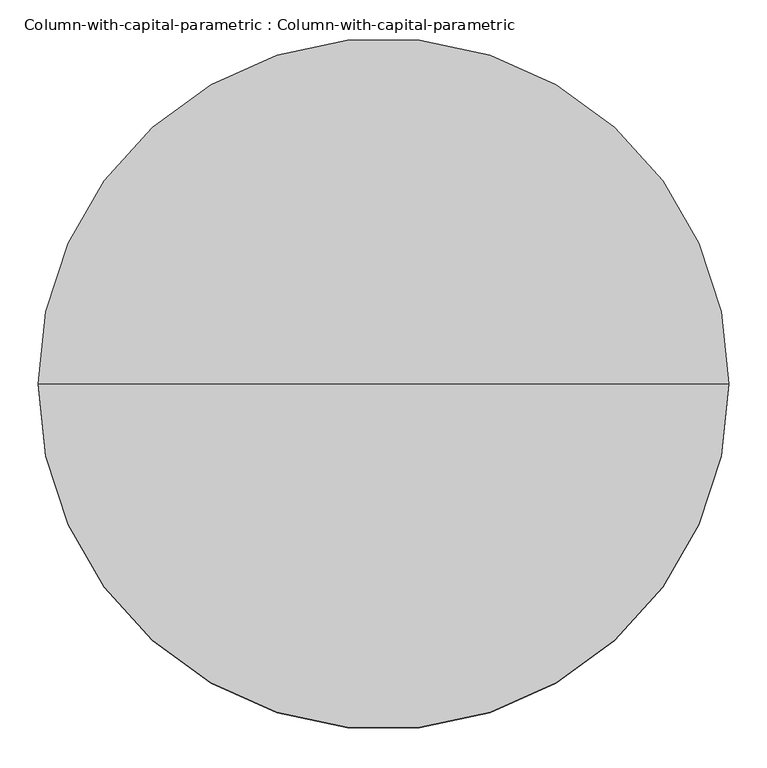
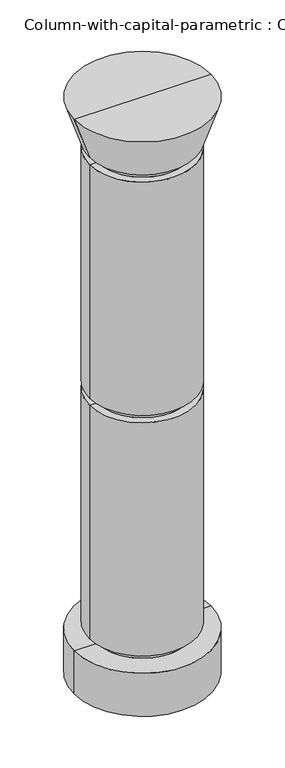
"""IFC4 building model written with IfcOpenShell, lengths in millimetres: column geometry, Column-with-capital-parametric : Column-with-capital-parametric."""

from ifc_helpers import new_model, si_unit, frame, origin, origin_with_axes, place, context, project, spatial, polyline, circle_curve, source, transform, mapped, element, save
from ifc_brep_helpers import plane_surface, cylinder_surface, revolved_surface, advanced_brep


def column_with_capital_parametric_column_with_capital_d26f2c8e(model_context):
    return source(origin(), model_context, "Body", "AdvancedBrep", [
        advanced_brep(
        [(-450.0, 0.0, 300.0), (450.0, 0.0, 300.0), (450.0, 0.0, 0.0), (-450.0, 0.0, 0.0), (0.0, 0.0, 0.0), (-300.0, 0.0, 300.0), (300.0, 0.0, 300.0), (-300.0, 0.0, 350.0), (300.0, 0.0, 350.0), (-350.0, 0.0, 350.0), (350.0, 0.0, 350.0), (-350.0, 0.0, 1975.0), (350.0, 0.0, 1975.0), (0.0, 0.0, 4000.0), (450.0, 0.0, 4000.0), (-450.0, 0.0, 4000.0), (350.0, 0.0, 3700.0), (-350.0, 0.0, 3700.0), (-300.0, 0.0, 3650.0), (300.0, 0.0, 3650.0), (350.0, 0.0, 3650.0), (-350.0, 0.0, 3650.0), (350.0, 0.0, 2025.0), (-350.0, 0.0, 2025.0), (-300.0, 0.0, 3700.0), (300.0, 0.0, 3700.0), (-300.0, 0.0, 1975.0), (300.0, 0.0, 1975.0), (-300.0, 0.0, 2025.0), (300.0, 0.0, 2025.0)],
        [
            (0, 1, circle_curve(frame((0.0, 0.0, 300.0), z_axis=(0.0, 0.0, -1.0), x_axis=(1.0, 0.0, 0.0)), 450.0)),
            (1, 2),
            (2, 3, circle_curve(origin_with_axes(), 450.0)),
            (3, 0),
            (2, 4),
            (4, 3),
            (2, 3, circle_curve(frame((0.0, 0.0, 0.0), z_axis=(0.0, 0.0, -1.0), x_axis=(1.0, 0.0, 0.0)), 450.0)),
            (1, 0, circle_curve(frame((0.0, 0.0, 300.0), z_axis=(0.0, 0.0, -1.0), x_axis=(1.0, 0.0, 0.0)), 450.0)),
            (5, 6, circle_curve(frame((0.0, 0.0, 300.0), z_axis=(0.0, 0.0, -1.0), x_axis=(1.0, 0.0, 0.0)), 300.0)),
            (6, 1),
            (0, 5),
            (6, 5, circle_curve(frame((0.0, 0.0, 300.0), z_axis=(0.0, 0.0, -1.0), x_axis=(1.0, 0.0, 0.0)), 300.0)),
            (7, 8, circle_curve(frame((0.0, 0.0, 350.0), z_axis=(0.0, 0.0, -1.0), x_axis=(1.0, 0.0, 0.0)), 300.0)),
            (8, 6),
            (5, 7),
            (8, 7, circle_curve(frame((0.0, 0.0, 350.0), z_axis=(0.0, 0.0, -1.0), x_axis=(1.0, 0.0, 0.0)), 300.0)),
            (9, 10, circle_curve(frame((0.0, 0.0, 350.0), z_axis=(0.0, 0.0, -1.0), x_axis=(1.0, 0.0, 0.0)), 350.0)),
            (10, 8),
            (7, 9),
            (10, 9, circle_curve(frame((0.0, 0.0, 350.0), z_axis=(0.0, 0.0, -1.0), x_axis=(1.0, 0.0, 0.0)), 350.0)),
            (11, 12, circle_curve(frame((0.0, 0.0, 1975.0), z_axis=(0.0, 0.0, -1.0), x_axis=(1.0, 0.0, 0.0)), 350.0)),
            (12, 10),
            (9, 11),
            (12, 11, circle_curve(frame((0.0, 0.0, 1975.0), z_axis=(0.0, 0.0, -1.0), x_axis=(1.0, 0.0, 0.0)), 350.0)),
            (13, 14),
            (14, 15, circle_curve(frame((0.0, 0.0, 4000.0), z_axis=(0.0, 0.0, 1.0), x_axis=(1.0, 0.0, 0.0)), 450.0)),
            (15, 13),
            (15, 14, circle_curve(frame((0.0, 0.0, 4000.0), z_axis=(0.0, 0.0, 1.0), x_axis=(1.0, 0.0, 0.0)), 450.0)),
            (14, 16),
            (16, 17, circle_curve(frame((0.0, 0.0, 3700.0), z_axis=(0.0, 0.0, 1.0), x_axis=(1.0, 0.0, 0.0)), 350.0)),
            (17, 15),
            (17, 16, circle_curve(frame((0.0, 0.0, 3700.0), z_axis=(0.0, 0.0, 1.0), x_axis=(1.0, 0.0, 0.0)), 350.0)),
            (18, 19, circle_curve(frame((0.0, 0.0, 3650.0), z_axis=(0.0, 0.0, -1.0), x_axis=(1.0, 0.0, 0.0)), 300.0)),
            (19, 20),
            (20, 21, circle_curve(frame((0.0, 0.0, 3650.0), z_axis=(0.0, 0.0, 1.0), x_axis=(1.0, 0.0, 0.0)), 350.0)),
            (21, 18),
            (20, 22),
            (22, 23, circle_curve(frame((0.0, 0.0, 2025.0), z_axis=(0.0, 0.0, 1.0), x_axis=(1.0, 0.0, 0.0)), 350.0)),
            (23, 21),
            (20, 21, circle_curve(frame((0.0, 0.0, 3650.0), z_axis=(0.0, 0.0, -1.0), x_axis=(1.0, 0.0, 0.0)), 350.0)),
            (23, 22, circle_curve(frame((0.0, 0.0, 2025.0), z_axis=(0.0, 0.0, 1.0), x_axis=(1.0, 0.0, 0.0)), 350.0)),
            (19, 18, circle_curve(frame((0.0, 0.0, 3650.0), z_axis=(0.0, 0.0, -1.0), x_axis=(1.0, 0.0, 0.0)), 300.0)),
            (24, 25, circle_curve(frame((0.0, 0.0, 3700.0), z_axis=(0.0, 0.0, -1.0), x_axis=(1.0, 0.0, 0.0)), 300.0)),
            (25, 19),
            (18, 24),
            (25, 24, circle_curve(frame((0.0, 0.0, 3700.0), z_axis=(0.0, 0.0, -1.0), x_axis=(1.0, 0.0, 0.0)), 300.0)),
            (16, 25),
            (24, 17),
            (26, 27, circle_curve(frame((0.0, 0.0, 1975.0), z_axis=(0.0, 0.0, -1.0), x_axis=(1.0, 0.0, 0.0)), 300.0)),
            (27, 12),
            (11, 26),
            (27, 26, circle_curve(frame((0.0, 0.0, 1975.0), z_axis=(0.0, 0.0, -1.0), x_axis=(1.0, 0.0, 0.0)), 300.0)),
            (28, 29, circle_curve(frame((0.0, 0.0, 2025.0), z_axis=(0.0, 0.0, -1.0), x_axis=(1.0, 0.0, 0.0)), 300.0)),
            (29, 27),
            (26, 28),
            (29, 28, circle_curve(frame((0.0, 0.0, 2025.0), z_axis=(0.0, 0.0, -1.0), x_axis=(1.0, 0.0, 0.0)), 300.0)),
            (22, 29),
            (28, 23),
        ],
        [
            cylinder_surface(frame((0.0, 0.0, 4203.0565088), z_axis=(0.0, 0.0, 1.0), x_axis=(1.0, 0.0, 0.0)), 450.0),
            plane_surface(frame((0.0, 0.0, 0.0), z_axis=(0.0, 0.0, -1.0), x_axis=(1.0, 0.0, 0.0))),
            plane_surface(frame((0.0, 0.0, 300.0), z_axis=(0.0, 0.0, 1.0), x_axis=(1.0, 0.0, 0.0))),
            cylinder_surface(frame((0.0, 0.0, 4203.0565088), z_axis=(0.0, 0.0, 1.0), x_axis=(1.0, 0.0, 0.0)), 300.0),
            plane_surface(frame((0.0, 0.0, 350.0), z_axis=(0.0, 0.0, -1.0), x_axis=(1.0, 0.0, 0.0))),
            cylinder_surface(frame((0.0, 0.0, 4203.0565088), z_axis=(0.0, 0.0, 1.0), x_axis=(1.0, 0.0, 0.0)), 350.0),
            plane_surface(frame((0.0, 0.0, 4000.0), z_axis=(0.0, 0.0, 1.0), x_axis=(1.0, 0.0, 0.0))),
            revolved_surface(polyline([(350.0, 0.0, 3700.0), (450.0, 0.0, 4000.0)]), (0.0, 0.0, 4203.0565088), (0.0, 0.0, 1.0)),
            plane_surface(frame((0.0, 0.0, 3650.0), z_axis=(0.0, 0.0, 1.0), x_axis=(1.0, 0.0, 0.0))),
            plane_surface(frame((0.0, 0.0, 3700.0), z_axis=(0.0, 0.0, -1.0), x_axis=(1.0, 0.0, 0.0))),
            plane_surface(frame((0.0, 0.0, 1975.0), z_axis=(0.0, 0.0, 1.0), x_axis=(1.0, 0.0, 0.0))),
            plane_surface(frame((0.0, 0.0, 2025.0), z_axis=(0.0, 0.0, -1.0), x_axis=(1.0, 0.0, 0.0))),
        ],
        [
            (0, [[1, 2, 3, 4]]),
            (1, [[-3, 5, 6]]),
            (1, [[7, -6, -5]]),
            (0, [[8, -4, -7, -2]]),
            (2, [[9, 10, -1, 11]]),
            (2, [[12, -11, -8, -10]]),
            (3, [[13, 14, -9, 15]]),
            (3, [[16, -15, -12, -14]]),
            (4, [[17, 18, -13, 19]]),
            (4, [[20, -19, -16, -18]]),
            (5, [[21, 22, -17, 23]]),
            (5, [[24, -23, -20, -22]]),
            (6, [[25, 26, 27]]),
            (6, [[-27, 28, -25]]),
            (7, [[-26, 29, 30, 31]]),
            (7, [[-28, -31, 32, -29]]),
            (8, [[33, 34, 35, 36]]),
            (5, [[-35, 37, 38, 39]]),
            (5, [[40, -39, 41, -37]]),
            (8, [[42, -36, -40, -34]]),
            (3, [[43, 44, -33, 45]]),
            (3, [[46, -45, -42, -44]]),
            (9, [[-30, 47, -43, 48]]),
            (9, [[-32, -48, -46, -47]]),
            (10, [[49, 50, -21, 51]]),
            (10, [[52, -51, -24, -50]]),
            (3, [[53, 54, -49, 55]]),
            (3, [[56, -55, -52, -54]]),
            (11, [[-38, 57, -53, 58]]),
            (11, [[-41, -58, -56, -57]]),
        ],
    ),
    ])


if __name__ == "__main__":
    model = new_model("IFC4")
    model_context = context("Model", 3, world=origin())
    ifc_project = project(units=[si_unit("LENGTHUNIT", "METRE", prefix="MILLI")], contexts=[model_context])
    site = spatial("IfcSite", under=ifc_project)
    building = spatial("IfcBuilding", under=site)
    placement = place(None, origin())
    column_with_capital_parametric_column_with_capital_shape = column_with_capital_parametric_column_with_capital_d26f2c8e(model_context)
    element("IfcColumn", 1, ObjectType="Column-with-capital-parametric : Column-with-capital-parametric", at=placement, inside=building, context=model_context, shape_type="MappedRepresentation", body=[
        mapped(column_with_capital_parametric_column_with_capital_shape, transform((0.0, 0.0, 0.0), x_axis=(1.0, 0.0, 0.0), y_axis=(0.0, 1.0, 0.0), z_axis=(0.0, 0.0, 1.0))),
    ])
    save(model, "model.ifc")

# Revit data of these elements
# Type "Column-with-capital-parametric : Column-with-capital-parametric"
#   Joint width = 50 mm
#   Diameter [instance default] = 600 mm
#   Capital height = 300 mm
#   Base height = 300 mm
# Element 1 (IfcColumn, "Column-with-capital-parametric : Column-with-capital-parametric")
#   Diameter = 900 mm
